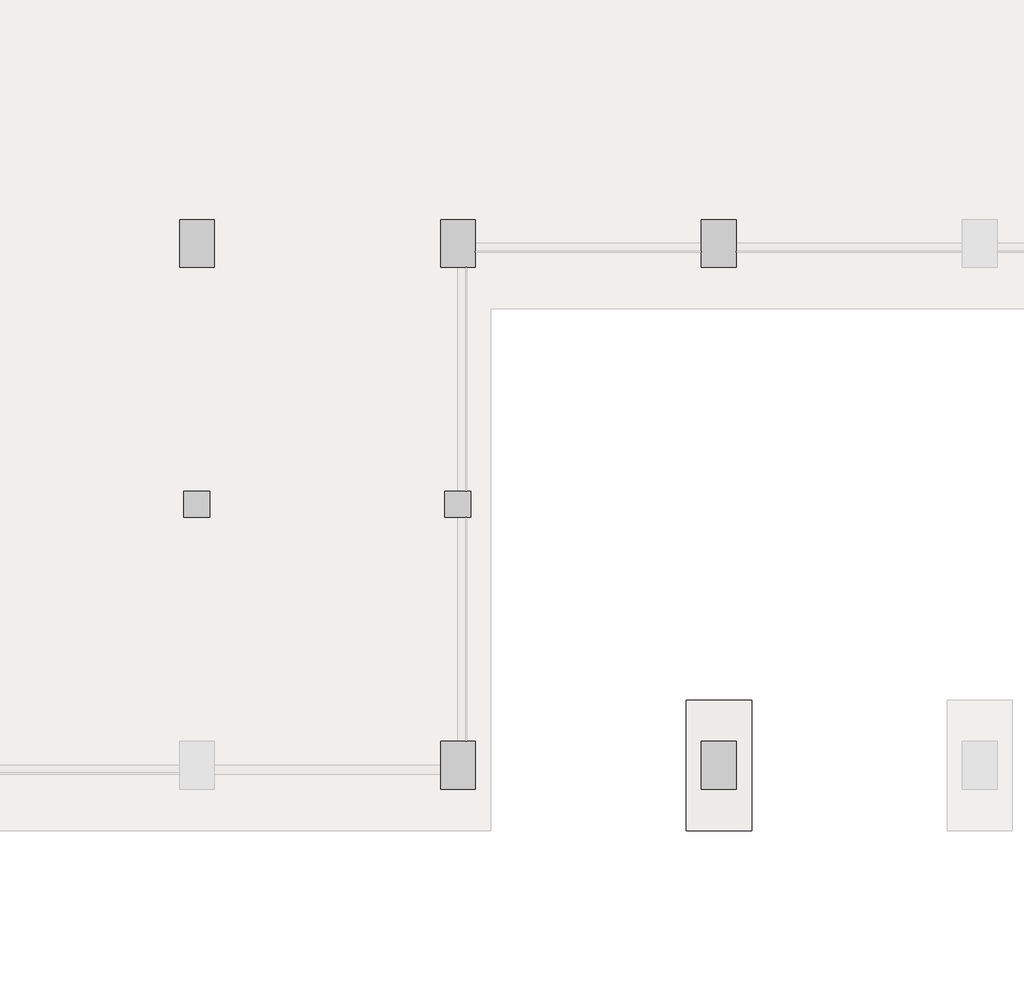
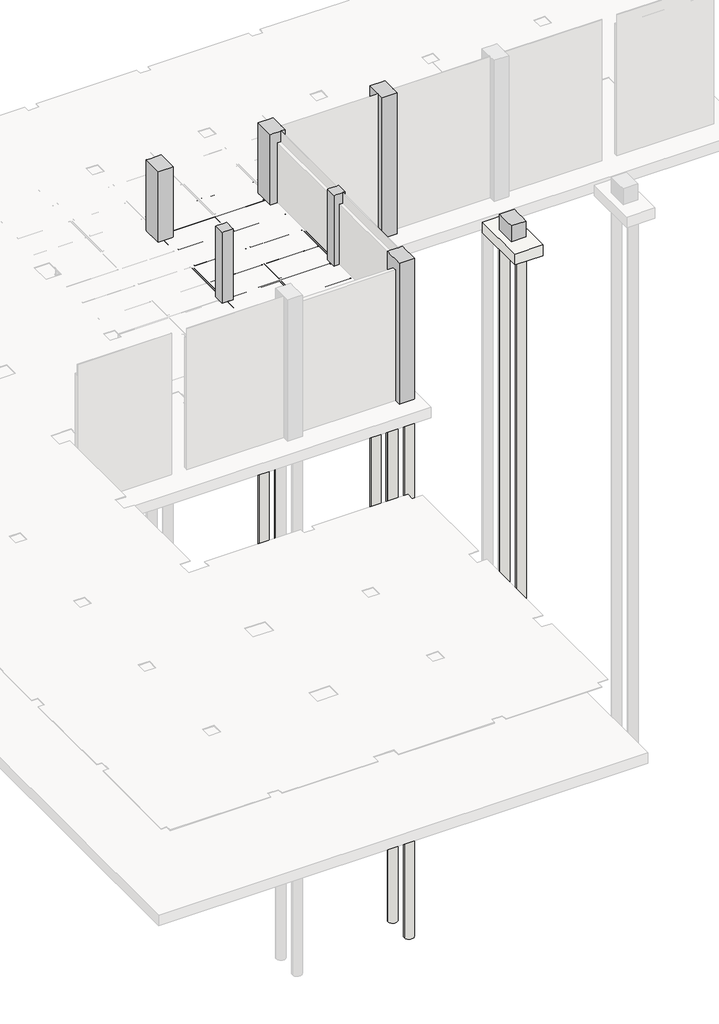
# Not in any storey, part 11 of 16: 24 beams, 9 slabs, 7 columns.
# Revit data of these elements (continued)
# Elements 2, 3, 4, 5, 6, 11, 12, 13, 14, 15, 16, 20, 21, 22, 23, 24 (IfcBeam, "Steel Framing_C_KS : H_SB_AR_S02_C-150x75x6.5x10_J1")
#   Structural Material = Steel, 45-345
#   Phase Created = New Construction
#   Materials on its faces: "Steel, 45-345"
# Elements 7, 9, 17, 18 (IfcBeam, "Steel Framing_H_KS : H_SB_AR_S02_H-400x200x8x13_BSG2")
#   Structural Material = Steel, 45-345
#   Phase Created = New Construction
#   Materials on its faces: "Steel, 45-345"
# Elements 10, 19 (IfcBeam, "Steel Framing_H_KS : H_SB_AR_S02_H-400x200x8x13_BSB1")
#   Structural Material = Steel, 45-345
#   Phase Created = New Construction
#   Materials on its faces: "Steel, 45-345"
# Elements 25, 26, 27, 28, 31 (IfcColumn, "RC_Column_Rectangular : H_SC_AR_S15_UG PED_Bit_800x1100_PD1")
#   Comments = ""
#   hec_material3 = none
#   hec_material2 = none
#   hec_material1 = none
#   Structural Material = 00_Concrete_Reinf. Conc.
#   Phase Created = New Construction
#   Materials on its faces: "00_Concrete_Reinf. Conc."
# Elements 29, 30 (IfcColumn, "RC_Column_Rectangular : H_SC_AR_S15_UG PED_Bit_600x600_BC1")
#   Comments = ""
#   hec_material3 = none
#   hec_material2 = none
#   hec_material1 = none
#   Structural Material = 00_Concrete_Reinf. Conc.
#   Phase Created = New Construction
#   Materials on its faces: "00_Concrete_Reinf. Conc."
# Element 32 (IfcSlab, "Foundation Rectangular (Non-Pile) : H_SF_AR_S18_Shallow Fdn_Bitumen_1500x3000xT600_F1")
#   Structural Material = 00_Concrete_Reinf. Conc.
#   Phase Created = New Construction
#   Materials on its faces: "00_Concrete_Reinf. Conc."
# Elements 33, 34 (IfcSlab, "PILE : H_SF_AR_S19_PHC Pile_Pre-boring_D500_L30")
#   Structural Material = Concrete, Precast
#   Phase Created = New Construction
#   Materials on its faces: "Concrete, Precast"
# Elements 35, 36, 37, 38, 39, 40 (IfcSlab, "PILE : H_SF_AR_S19_PHC Pile_Pre-boring_D500_L30")
#   Structural Material = none
#   Phase Created = New Construction
# Materials
#   "Steel, 45-345": class "Metal", colour RGB 189 187 185, transparency 0, Description = "Steel 345 MPa", Cost = 0
#   "00_Concrete_Reinf. Conc.": class "Concrete", colour RGB 176 176 176, transparency 0, Description = "Reinf. Conc.", Cost = 0, Image = Concrete.Cast-In-Place.Flat.Polished.Grey.jpg
#   "Concrete, Precast": class "Concrete", colour RGB 115 116 108, transparency 0, Description = "Precast concrete", Cost = 0
